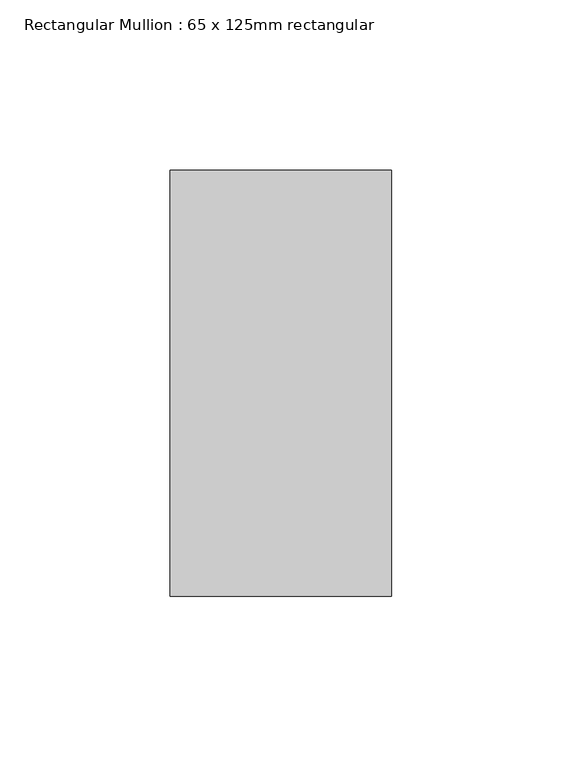
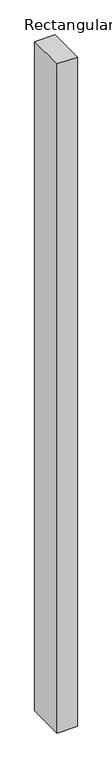
"""IFC4 building model written with IfcOpenShell, lengths in millimetres: member geometry, Rectangular Mullion : 65 x 125mm rectangular."""

from ifc_helpers import new_model, si_unit, frame, origin, place, context, project, spatial, polyline, outline, extrude, source, transform, mapped, element, save


def rectangular_mullion_65_x_125mm_rectangular_478791df(model_context):
    return source(origin(), model_context, "Body", "SweptSolid", [
        extrude(outline(polyline([(0.0, 62.5), (0.0, -62.5), (-65.0, -62.5), (-65.0, 62.5), (0.0, 62.5)])), frame((0.0, 0.0, -2277.3304137), z_axis=(0.0, 0.0, 1.0), x_axis=(1.0, 0.0, 0.0)), (0.0, 0.0, 1.0), 2277.3304137),
    ])


if __name__ == "__main__":
    model = new_model("IFC4")
    model_context = context("Model", 3, world=origin())
    ifc_project = project(units=[si_unit("LENGTHUNIT", "METRE", prefix="MILLI")], contexts=[model_context])
    site = spatial("IfcSite", under=ifc_project)
    building = spatial("IfcBuilding", under=site)
    placement = place(None, origin())
    rectangular_mullion_65_x_125mm_rectangular_shape = rectangular_mullion_65_x_125mm_rectangular_478791df(model_context)
    element("IfcMember", 1, ObjectType="Rectangular Mullion : 65 x 125mm rectangular", at=placement, inside=building, context=model_context, shape_type="MappedRepresentation", body=[
        mapped(rectangular_mullion_65_x_125mm_rectangular_shape, transform((0.0, 0.0, 0.0), x_axis=(1.0, 0.0, 0.0), y_axis=(0.0, 1.0, 0.0), z_axis=(0.0, 0.0, 1.0))),
    ])
    save(model, "model.ifc")

# Revit data of these elements
# Type "Rectangular Mullion : 65 x 125mm rectangular"
#   built-in parameter 1007304 = 0.410105 (stored number, unit not read)
#   built-in parameter 1007301 = 0.106627 (stored number, unit not read)
#   built-in parameter 1007300 = 0.106627 (stored number, unit not read)
# Element 1 (IfcMember, "Rectangular Mullion : 65 x 125mm rectangular")
#   Materials on its faces: "Aluminum"
# Materials
#   "Aluminum": class "Metal", colour RGB 244 245 246, transparency 0, Description = "Aluminum 6061", Cost = 0
